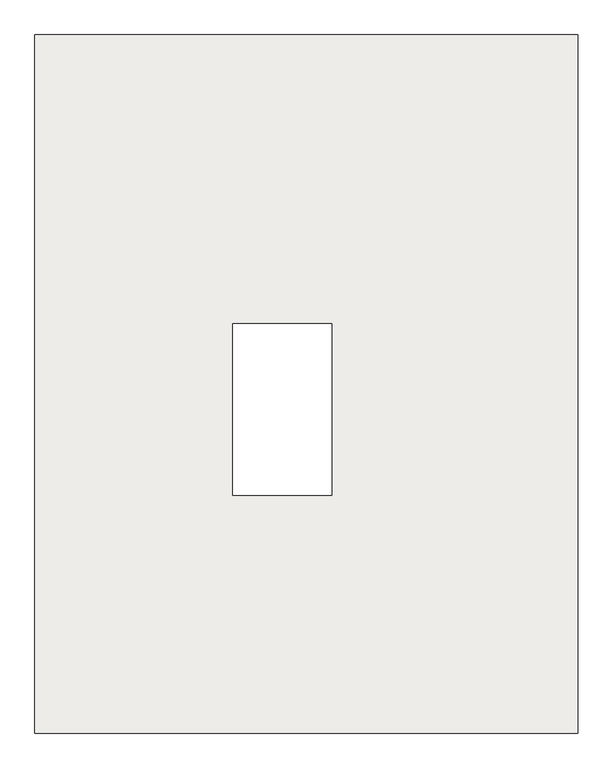
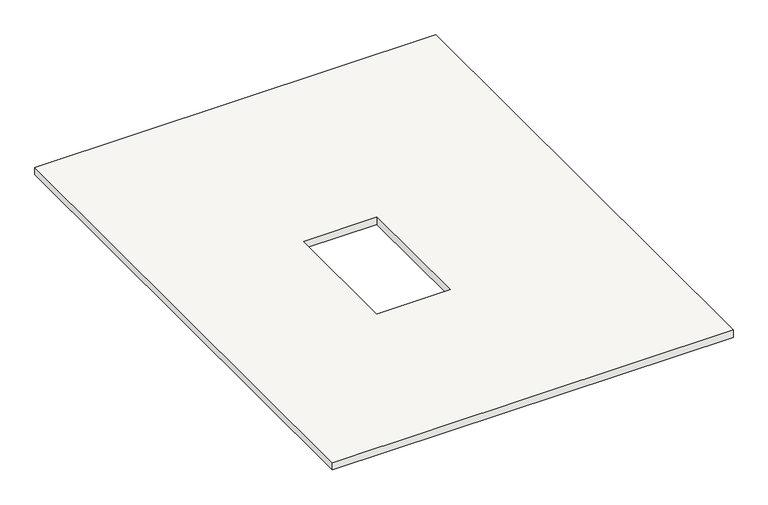
"""IFC4 building model written with IfcOpenShell, lengths in millimetres: slab geometry, Holzdecke."""

import ifcopenshell
import ifcopenshell.guid

model = None  # the IFC model being written
_history = None  # IfcOwnerHistory: only IFC2X3 demands one
_inside = {}  # id of a spatial element -> (the spatial element, [elements in it])
_under = {}  # id of a project, library or spatial element -> (it, [spatial elements below it])
_declared = {}  # id of a project -> (the project, [libraries it declares])
_typed = {}  # id of a type object -> (the type object, [elements of that type])
_made_of = {}  # id of a material, layer set ... -> (it, [elements and type objects made of it])


def new_model(schema):
    """Start an empty IFC model of exactly this schema.

    Asked for "IFC4X3", IfcOpenShell would pick the latest addendum, in which some entities
    have other attributes; the version numbers below select the first issue.
    IFC2X3 requires an IfcOwnerHistory on every rooted entity: one is made here for all.
    """
    global model, _history
    if schema == "IFC4X3":
        model = ifcopenshell.file(schema_version=(4, 3, 0, 0))
    else:
        model = ifcopenshell.file(schema=schema)
    _inside.clear()
    _under.clear()
    _declared.clear()
    _typed.clear()
    _made_of.clear()
    _history = None
    if model.schema == "IFC2X3":
        org = make("IfcOrganization", Name="unknown")
        user = make(
            "IfcPersonAndOrganization",
            ThePerson=make("IfcPerson", FamilyName="unknown"),
            TheOrganization=org,
        )
        app = make(
            "IfcApplication",
            ApplicationDeveloper=org,
            Version="unknown",
            ApplicationFullName="unknown",
            ApplicationIdentifier="unknown",
        )
        _history = make(
            "IfcOwnerHistory",
            OwningUser=user,
            OwningApplication=app,
            ChangeAction="ADDED",
            CreationDate=0,
        )
    return model


def make(cls, **values):
    """One entity of the class cls with the attributes given. An attribute that is None is left unset."""
    return model.create_entity(
        cls, **{name: value for name, value in values.items() if value is not None}
    )


def rooted(cls, **values):
    """An entity with a GlobalId (a new one), such as an element, a storey or a relation."""
    return make(cls, GlobalId=ifcopenshell.guid.new(), OwnerHistory=_history, **values)


def si_unit(unit_type, name, prefix=None):
    """IfcSIUnit, for example si_unit("LENGTHUNIT", "METRE", prefix="MILLI")."""
    return make("IfcSIUnit", UnitType=unit_type, Prefix=prefix, Name=name)


def assignment(units):
    """IfcUnitAssignment: the units of a project."""
    return None if units is None else make("IfcUnitAssignment", Units=units)


def point(xyz):
    """IfcCartesianPoint."""
    return None if xyz is None else make("IfcCartesianPoint", Coordinates=xyz)


def direction(xyz):
    """IfcDirection."""
    return None if xyz is None else make("IfcDirection", DirectionRatios=xyz)


def frame(location, z_axis=None, x_axis=None):
    """IfcAxis2Placement3D, a coordinate frame: its origin and axes. An axis left out is left unset."""
    return make(
        "IfcAxis2Placement3D",
        Location=point(location),
        Axis=direction(z_axis),
        RefDirection=direction(x_axis),
    )


def origin():
    """The frame at (0, 0, 0) with its axes left unset."""
    return frame((0.0, 0.0, 0.0))


def origin_with_axes():
    """The frame at (0, 0, 0) with the z axis (0, 0, 1) and the x axis (1, 0, 0) written out."""
    return frame((0.0, 0.0, 0.0), z_axis=(0.0, 0.0, 1.0), x_axis=(1.0, 0.0, 0.0))


def place(relative_to, where):
    """IfcLocalPlacement: puts the frame where relative to a parent placement (None: the world)."""
    return make(
        "IfcLocalPlacement", PlacementRelTo=relative_to, RelativePlacement=where
    )


def context(
    kind, dimensions, precision=None, world=None, true_north=None, identifier=None
):
    """IfcGeometricRepresentationContext, for example the 3D "Model" context."""
    return make(
        "IfcGeometricRepresentationContext",
        ContextIdentifier=identifier,
        ContextType=kind,
        CoordinateSpaceDimension=dimensions,
        Precision=precision,
        WorldCoordinateSystem=world,
        TrueNorth=true_north,
    )


def project(units=None, contexts=None):
    """IfcProject with its units and contexts."""
    return rooted(
        "IfcProject",
        Name="project",
        RepresentationContexts=contexts,
        UnitsInContext=assignment(units),
    )


def spatial(cls, under=None, at=None, **own):
    """A site, building, storey or space (cls), placed at a placement, below another one or the project."""
    s = rooted(cls, ObjectPlacement=at, **own)
    if under is not None:
        _under.setdefault(under.id(), (under, []))[1].append(s)
    return s


def polyline(points):
    """IfcPolyline through the points."""
    return make("IfcPolyline", Points=[point(p) for p in points])


def outline(outer, holes=None, kind="AREA"):
    """IfcArbitraryClosedProfileDef: a profile drawn as a closed curve; with holes, ...WithVoids."""
    if holes is None:
        return make("IfcArbitraryClosedProfileDef", ProfileType=kind, OuterCurve=outer)
    return make(
        "IfcArbitraryProfileDefWithVoids",
        ProfileType=kind,
        OuterCurve=outer,
        InnerCurves=holes,
    )


def extrude(swept, where, along, depth):
    """IfcExtrudedAreaSolid: the profile swept, set in the frame where, extruded along a direction by depth."""
    return make(
        "IfcExtrudedAreaSolid",
        SweptArea=swept,
        Position=where,
        ExtrudedDirection=direction(along),
        Depth=depth,
    )


def shape(context_of_items, identifier, shape_type, items):
    """IfcShapeRepresentation: the items that make up one representation, for example the "Body"."""
    return make(
        "IfcShapeRepresentation",
        ContextOfItems=context_of_items,
        RepresentationIdentifier=identifier,
        RepresentationType=shape_type,
        Items=items,
    )


def source(mapping_origin, context_of_items, identifier, shape_type, items):
    """IfcRepresentationMap: a shape defined once, which mapped items show again and again."""
    return make(
        "IfcRepresentationMap",
        MappingOrigin=mapping_origin,
        MappedRepresentation=shape(context_of_items, identifier, shape_type, items),
    )


def transform(
    local_origin,
    x_axis=None,
    y_axis=None,
    z_axis=None,
    scale=None,
    scale2=None,
    scale3=None,
    uniform=True,
):
    """IfcCartesianTransformationOperator3D, or its non-uniform kind. x_axis, y_axis, z_axis: its Axis1, 2, 3."""
    if uniform:
        return make(
            "IfcCartesianTransformationOperator3D",
            Axis1=direction(x_axis),
            Axis2=direction(y_axis),
            LocalOrigin=point(local_origin),
            Scale=scale,
            Axis3=direction(z_axis),
        )
    return make(
        "IfcCartesianTransformationOperator3DnonUniform",
        Axis1=direction(x_axis),
        Axis2=direction(y_axis),
        LocalOrigin=point(local_origin),
        Scale=scale,
        Axis3=direction(z_axis),
        Scale2=scale2,
        Scale3=scale3,
    )


def mapped(mapping_source, mapping_target):
    """IfcMappedItem: shows the shape of a source again, moved by a transform."""
    return make(
        "IfcMappedItem", MappingSource=mapping_source, MappingTarget=mapping_target
    )


def made_of(thing, what):
    """Note that an element or type object is made of a material, layer set ...; save() writes the relation."""
    if what is not None:
        _made_of.setdefault(what.id(), (what, []))[1].append(thing)
    return thing


def element(
    cls,
    number,
    at=None,
    inside=None,
    cuts=None,
    type_object=None,
    material=None,
    context=None,
    identifier="Body",
    shape_type=None,
    held_by="IfcProductDefinitionShape",
    body=None,
    shapes=None,
    **own,
):
    """One element of the class cls, such as IfcWall. Its Tag is "e" and its number.

    at: its placement. inside: the storey or other place that contains it. cuts: it is an
    opening in that element (IfcRelVoidsElement). A single representation is given by context,
    identifier, shape_type and body (its items); several are given by shapes. held_by: the class
    of the entity that holds the representations. save() writes the other relations.
    """
    e = rooted(cls, Tag="e%d" % number, ObjectPlacement=at, **own)
    if body is not None:
        shapes = [shape(context, identifier, shape_type, body)]
    if shapes is not None:
        e.Representation = make(held_by, Representations=shapes)
    if inside is not None:
        _inside.setdefault(inside.id(), (inside, []))[1].append(e)
    if cuts is not None:
        rooted(
            "IfcRelVoidsElement", RelatingBuildingElement=cuts, RelatedOpeningElement=e
        )
    if type_object is not None:
        _typed.setdefault(type_object.id(), (type_object, []))[1].append(e)
    return made_of(e, material)


def aggregate(whole, parts):
    """IfcRelAggregates: a whole, such as a stair, and the parts it consists of."""
    return rooted("IfcRelAggregates", RelatingObject=whole, RelatedObjects=parts)


def save(model, path):
    """Write the relations noted so far, then the file.

    IfcRelAggregates (storeys below a building ...), IfcRelContainedInSpatialStructure (elements
    in a storey), IfcRelDefinesByType, IfcRelAssociatesMaterial and IfcRelDeclares: one each for
    every whole, place, type object, material and project.
    """
    for whole, parts in _under.values():
        aggregate(whole, parts)
    for where, things in _inside.values():
        rooted(
            "IfcRelContainedInSpatialStructure",
            RelatedElements=things,
            RelatingStructure=where,
        )
    for kind, things in _typed.values():
        rooted("IfcRelDefinesByType", RelatedObjects=things, RelatingType=kind)
    for what, things in _made_of.values():
        rooted("IfcRelAssociatesMaterial", RelatedObjects=things, RelatingMaterial=what)
    for by, libraries in _declared.values():
        rooted("IfcRelDeclares", RelatingContext=by, RelatedDefinitions=libraries)
    model.write(path)


def slab_2880fc09(model_context):
    return source(origin(), model_context, "Body", "SweptSolid", [
        extrude(outline(polyline([(0.0, 0.0), (0.0, 18002.8619019), (14000.0, 18002.8619019), (14000.0, 0.0), (0.0, 0.0)]), holes=[polyline([(7650.0, 6132.8619019), (7650.0, 10552.8619019), (5100.0, 10552.8619019), (5100.0000123, 6134.7780147), (7650.0, 6132.8619019)])]), origin_with_axes(), (0.0, 0.0, 1.0), 270.0),
    ])


if __name__ == "__main__":
    model = new_model("IFC4")
    model_context = context("Model", 3, world=origin())
    ifc_project = project(units=[si_unit("LENGTHUNIT", "METRE", prefix="MILLI")], contexts=[model_context])
    site = spatial("IfcSite", under=ifc_project)
    building = spatial("IfcBuilding", under=site)
    placement = place(None, origin())
    slab_shape = slab_2880fc09(model_context)
    element("IfcSlab", 1, ObjectType="Holzdecke", at=placement, inside=building, context=model_context, shape_type="MappedRepresentation", body=[
        mapped(slab_shape, transform((0.0, 0.0, 0.0), x_axis=(1.0, 0.0, 0.0), y_axis=(0.0, 1.0, 0.0), z_axis=(0.0, 0.0, 1.0))),
    ])
    save(model, "model.ifc")

# Revit data of these elements
# Element 1 (IfcSlab, "Holzdecke")
#   Materials on its faces: "holzschalung"
# Materials
#   "holzschalung": class "Unassigned", colour RGB 128 128 128, transparency 0
